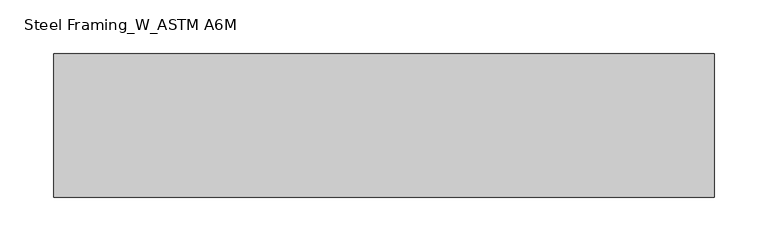
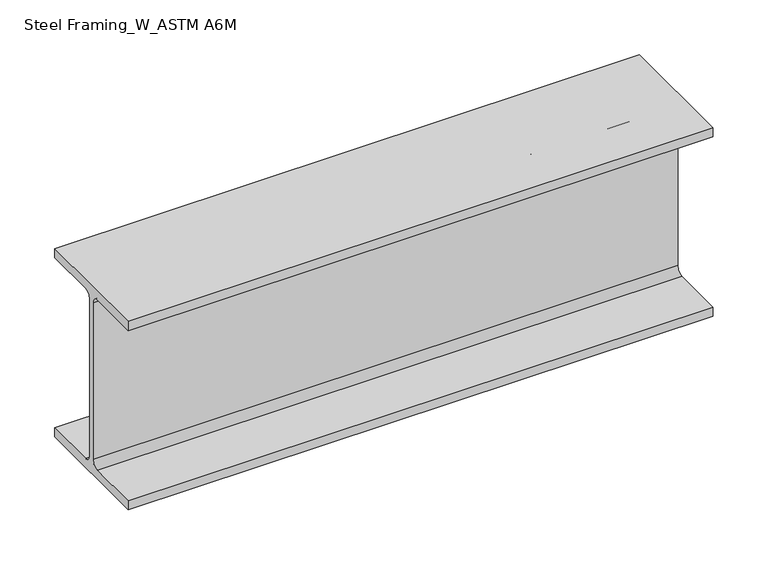
"""IFC4 building model written with IfcOpenShell, lengths in millimetres: beam geometry, Steel Framing_W_ASTM A6M : H_SB_AR_S02_W200x31.3_B6."""

from ifc_helpers import new_model, si_unit, point, frame, frame_2d, origin, place, context, project, spatial, polyline, circle_curve, trimmed, segment, composite_curve, outline, extrude, source, transform, mapped, element, save


def steel_framing_w_astm_a6m_676d03db(model_context):
    return source(origin(), model_context, "Body", "SweptSolid", [
        extrude(outline(composite_curve([segment(polyline([(67.0, -94.8), (67.0, -105.0), (-67.0, -105.0), (-67.0, -94.8), (-10.775, -94.8)]), True, "CONTINUOUS"), segment(trimmed(circle_curve(frame_2d((-10.775, -87.2)), 7.6), [point((-10.775, -94.8))], [point((-3.175, -87.2))], True, "CARTESIAN"), True, "CONTINUOUS"), segment(polyline([(-3.175, -87.2), (-3.175, 87.2)]), True, "CONTINUOUS"), segment(trimmed(circle_curve(frame_2d((-10.775, 87.2)), 7.6), [point((-3.175, 87.2))], [point((-10.775, 94.8))], True, "CARTESIAN"), True, "CONTINUOUS"), segment(polyline([(-10.775, 94.8), (-67.0, 94.8), (-67.0, 105.0), (67.0, 105.0), (67.0, 94.8), (10.775, 94.8)]), True, "CONTINUOUS"), segment(trimmed(circle_curve(frame_2d((10.775, 87.2)), 7.6), [point((10.775, 94.8))], [point((3.175, 87.2))], True, "CARTESIAN"), True, "CONTINUOUS"), segment(polyline([(3.175, 87.2), (3.175, -87.2)]), True, "CONTINUOUS"), segment(trimmed(circle_curve(frame_2d((10.775, -87.2)), 7.6), [point((3.175, -87.2))], [point((10.775, -94.8))], True, "CARTESIAN"), True, "CONTINUOUS"), segment(polyline([(10.775, -94.8), (67.0, -94.8)]), True, "CONTINUOUS")], self_intersect=False)), frame((-345.3, 0.0, 0.0), z_axis=(1.0, 0.0, 0.0), x_axis=(0.0, 1.0, 0.0)), (0.0, 0.0, 1.0), 616.6),
    ])


if __name__ == "__main__":
    model = new_model("IFC4")
    model_context = context("Model", 3, world=origin())
    ifc_project = project(units=[si_unit("LENGTHUNIT", "METRE", prefix="MILLI")], contexts=[model_context])
    site = spatial("IfcSite", under=ifc_project)
    building = spatial("IfcBuilding", under=site)
    placement = place(None, origin())
    steel_framing_w_astm_a6m_shape = steel_framing_w_astm_a6m_676d03db(model_context)
    element("IfcBeam", 1, ObjectType="Steel Framing_W_ASTM A6M : H_SB_AR_S02_W200x31.3_B6", at=placement, inside=building, context=model_context, shape_type="MappedRepresentation", body=[
        mapped(steel_framing_w_astm_a6m_shape, transform((0.0, 0.0, 0.0), x_axis=(1.0, 0.0, 0.0), y_axis=(0.0, 1.0, 0.0), z_axis=(0.0, 0.0, 1.0))),
    ])
    save(model, "model.ifc")

# Revit data of these elements
# Type "Steel Framing_W_ASTM A6M : H_SB_AR_S02_W200x31.3_B6"
#   Type Mark = "B6"
#   Section Name Key = "W8x21"
#   Width = 13.4 cm
#   Web Thickness = 0.635 cm
#   Web Fillet = 0.76 cm
#   Warping Constant = 40800.0 cm⁶
#   Torsional Moment of Inertia = 11.70 cm⁴
#   Section Area = 39.7 cm²
#   Plastic Modulus weak axis = 93.2 cm³
#   Plastic Modulus strong axis = 334.0 cm³
#   Perimeter = 0.93 m²/m
#   Nominal Weight = 31.30 kgf/m
#   Moment of Inertia weak axis = 407.00 cm⁴
#   Moment of Inertia strong axis = 3130.00 cm⁴
#   Height = 21.0 cm
#   Flange Thickness = 1.02 cm
#   Elastic Modulus weak axis = 60.8 cm³
#   Elastic Modulus strong axis = 298.0 cm³
#   Centroid Vertical = 10.5 cm
#   Centroid Horizontal = 6.7 cm
#   Length [instance default] = 1500 mm
#   Structural Material [instance default] = Steel, 45-345
#   Bolt Spacing = 0
#   Assembly Code = ""
# Element 1 (IfcBeam, "Steel Framing_W_ASTM A6M : H_SB_AR_S02_W200x31.3_B6")
#   Materials on its faces: "Steel, 45-345"
# Materials
#   "Steel, 45-345": class "Metal", colour RGB 189 187 185, transparency 0, Description = "Steel 345 MPa", Cost = 0
